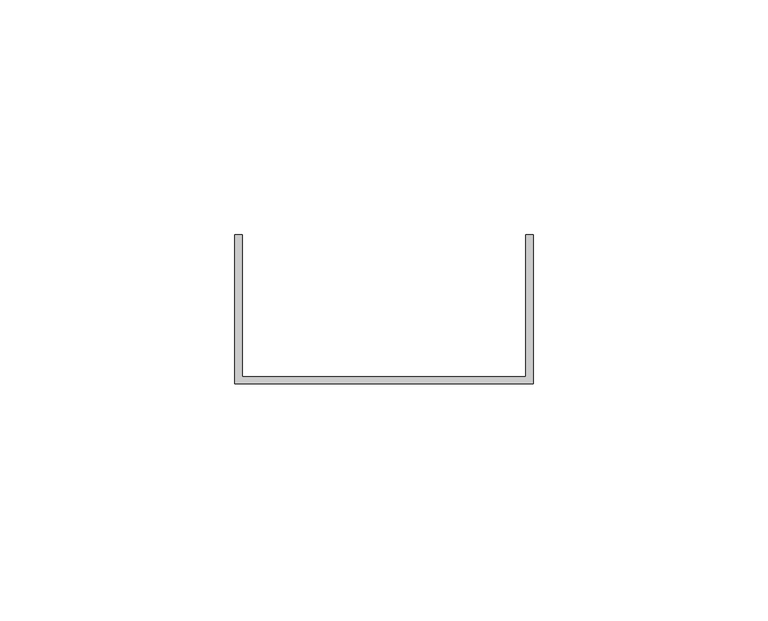
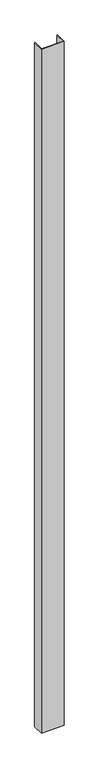
"""IFC4 building model written with IfcOpenShell, lengths in millimetres: proxy geometry, Generic Models 7:Generic Models 1:3:Generic Models 1:3 : Generic Models 7:Generic Models 1:305549:3:Generic Models 1:3:Generic Models 1:3 : Generic Models 7:Generic Models 1:305549:3 : Generic Models 7:Generic Models 1:3:Generic Models 1:3 : Generic Models 7:Generic Models 1:305549:301244:12 : Generic Models 7:Generic Models 1:3:Generic Models 1:3 : Generic Models 7:Generic Models 1:305549:3:Generic Models 1:3:Generic Models 1:3 : Generic Models 7:Generic Models 1:305549:3 : Generic Models 7:Generic Models 1:3:Generic Models 1:3 : Generic Models 7:Generic Models 1:305549:301244:308848."""

from ifc_helpers import new_model, si_unit, frame, origin, place, context, project, spatial, polyline, outline, extrude, source, transform, mapped, element, save


def generic_models_1ae3f7b5(model_context):
    return source(origin(), model_context, "Body", "SweptSolid", [
        extrude(outline(polyline([(579320.411724, -579000.6913841), (579320.411724, -578968.9413841), (579321.999224, -578968.9413841), (579321.999224, -578999.1038841), (579382.3242239, -578999.1038841), (579382.3242239, -578968.9413841), (579383.9117239, -578968.9413841), (579383.9117239, -579000.6913841), (579320.411724, -579000.6913841)])), frame((0.0, 0.0, 4133.81326), z_axis=(0.0, 0.0, 1.0), x_axis=(1.0, 0.0, 0.0)), (0.0, 0.0, 1.0), 2000.28674),
    ])


if __name__ == "__main__":
    model = new_model("IFC4")
    model_context = context("Model", 3, world=origin())
    ifc_project = project(units=[si_unit("LENGTHUNIT", "METRE", prefix="MILLI")], contexts=[model_context])
    site = spatial("IfcSite", under=ifc_project)
    building = spatial("IfcBuilding", under=site)
    placement = place(None, origin())
    generic_models_shape = generic_models_1ae3f7b5(model_context)
    element("IfcBuildingElementProxy", 1, Name="Generic Models 7:Generic Models 1:3:Generic Models 1:3 : Generic Models 7:Generic Models 1:305549:3:Generic Models 1:3:Generic Models 1:3 : Generic Models 7:Generic Models 1:305549:3 : Generic Models 7:Generic Models 1:3:Generic Models 1:3 : Generic Models 7:Generic Models 1:305549:301244:12 : Generic Models 7:Generic Models 1:3:Generic Models 1:3 : Generic Models 7:Generic Models 1:305549:3:Generic Models 1:3:Generic Models 1:3 : Generic Models 7:Generic Models 1:305549:3 : Generic Models 7:Generic Models 1:3:Generic Models 1:3 : Generic Models 7:Generic Models 1:305549:301244:308848", ObjectType="Generic Models 7:Generic Models 1:3:Generic Models 1:3 : Generic Models 7:Generic Models 1:305549:3:Generic Models 1:3:Generic Models 1:3 : Generic Models 7:Generic Models 1:305549:3 : Generic Models 7:Generic Models 1:3:Generic Models 1:3 : Generic Models 7:Generic Models 1:305549:301244:12 : Generic Models 7:Generic Models 1:3:Generic Models 1:3 : Generic Models 7:Generic Models 1:305549:3:Generic Models 1:3:Generic Models 1:3 : Generic Models 7:Generic Models 1:305549:3 : Generic Models 7:Generic Models 1:3:Generic Models 1:3 : Generic Models 7:Generic Models 1:305549:301244:308848", at=placement, inside=building, context=model_context, shape_type="MappedRepresentation", body=[
        mapped(generic_models_shape, transform((0.0, 0.0, 0.0), x_axis=(1.0, 0.0, 0.0), y_axis=(0.0, 1.0, 0.0), z_axis=(0.0, 0.0, 1.0))),
    ])
    save(model, "model.ifc")

# Revit data of these elements
# Type "Generic Models 7:Generic Models 1:3:Generic Models 1:3 : Generic Models 7:Generic Models 1:305549:3:Generic Models 1:3:Generic Models 1:3 : Generic Models 7:Generic Models 1:305549:3 : Generic Models 7:Generic Models 1:3:Generic Models 1:3 : Generic Models 7:Generic Models 1:305549:301244:12 : Generic Models 7:Generic Models 1:3:Generic Models 1:3 : Generic Models 7:Generic Models 1:305549:3:Generic Models 1:3:Generic Models 1:3 : Generic Models 7:Generic Models 1:305549:3 : Generic Models 7:Generic Models 1:3:Generic Models 1:3 : Generic Models 7:Generic Models 1:305549:301244:308848"
#   NameOverride = "Generic Models 7:Generic Models 1:3:Generic Models 1:3 : Generic Models 7:Generic Models 1:305549:3:Generic Models 1:3:Generic Models 1:3 : Generic Models 7:Generic Models 1:305549:3 : Generic Models 7:Generic Models 1:3:Generic Models 1:3 : Generic Models 7:Generic Models 1:305549:301244:308848"
#   ObjectTypeOverride = "Generic Models 1:3:Generic Models 1:3 : Generic Models 7:Generic Models 1:305549:3 : Generic Models 7:Generic Models 1:3:Generic Models 1:3 : Generic Models 7:Generic Models 1:305549:301244"
#   Reference = "Generic Models 1"
#   Tag = "308848"
# Element 1 (IfcBuildingElementProxy, "Generic Models 7:Generic Models 1:3:Generic Models 1:3 : Generic Models 7:Generic Models 1:305549:3:Generic Models 1:3:Generic Models 1:3 : Generic Models 7:Generic Models 1:305549:3 : Generic Models 7:Generic Models 1:3:Generic Models 1:3 : Generic Models 7:Generic Models 1:305549:301244:12 : Generic Models 7:Generic Models 1:3:Generic Models 1:3 : Generic Models 7:Generic Models 1:305549:3:Generic Models 1:3:Generic Models 1:3 : Generic Models 7:Generic Models 1:305549:3 : Generic Models 7:Generic Models 1:3:Generic Models 1:3 : Generic Models 7:Generic Models 1:305549:301244:308848")
#   Materials on its faces: "GALVANIZED U-CHANNEL (250T125-33)"
# Materials
#   "GALVANIZED U-CHANNEL (250T125-33)": class "Unassigned", colour RGB 202 201 200, transparency 0, Keynote = "M05451300.02", Cost = 0
